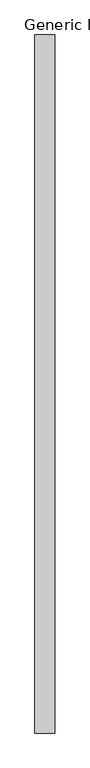
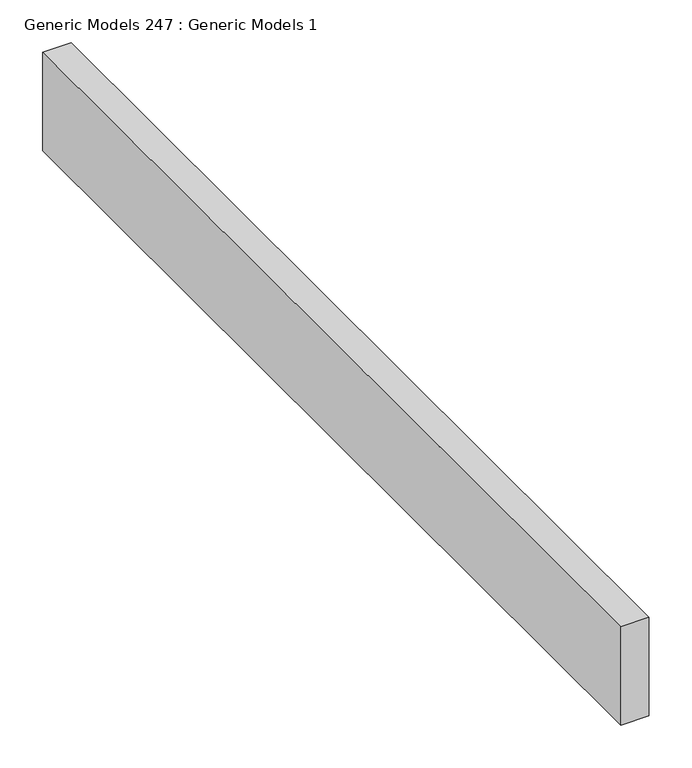
"""IFC4 building model written with IfcOpenShell, lengths in millimetres: proxy geometry, Generic Models 247 : Generic Models 1."""

from ifc_helpers import new_model, si_unit, frame, origin, place, context, project, spatial, polyline, outline, extrude, source, transform, mapped, element, save


def generic_models_247_generic_models_1_75e2395a(model_context):
    return source(origin(), model_context, "Body", "SweptSolid", [
        extrude(outline(polyline([(2172.2490992, -21510.2473745), (2134.1490992, -21510.2473745), (2134.1490992, -20164.0473745), (2172.2490992, -20164.0473745), (2172.2490992, -21510.2473745)])), frame((0.0, 0.0, 126814.0999329), z_axis=(0.0, 0.0, 1.0), x_axis=(1.0, 0.0, 0.0)), (0.0, 0.0, 1.0), 139.7),
    ])


if __name__ == "__main__":
    model = new_model("IFC4")
    model_context = context("Model", 3, world=origin())
    ifc_project = project(units=[si_unit("LENGTHUNIT", "METRE", prefix="MILLI")], contexts=[model_context])
    site = spatial("IfcSite", under=ifc_project)
    building = spatial("IfcBuilding", under=site)
    placement = place(None, origin())
    generic_models_247_generic_models_1_shape = generic_models_247_generic_models_1_75e2395a(model_context)
    element("IfcBuildingElementProxy", 1, Name="Generic Models 247 : Generic Models 1", ObjectType="Generic Models 247 : Generic Models 1", at=placement, inside=building, context=model_context, shape_type="MappedRepresentation", body=[
        mapped(generic_models_247_generic_models_1_shape, transform((0.0, 0.0, 0.0), x_axis=(1.0, 0.0, 0.0), y_axis=(0.0, 1.0, 0.0), z_axis=(0.0, 0.0, 1.0))),
    ])
    save(model, "model.ifc")

# Revit data of these elements
# Element 1 (IfcBuildingElementProxy, "Generic Models 247 : Generic Models 1")
#   Materials on its faces: "_STRUCTURAL MEMBER (SEE STRUCT. DWGS)"
# Materials
#   "_STRUCTURAL MEMBER (SEE STRUCT. DWGS)": class "Generic", colour RGB 209 182 141, transparency 0, Cost = 0
